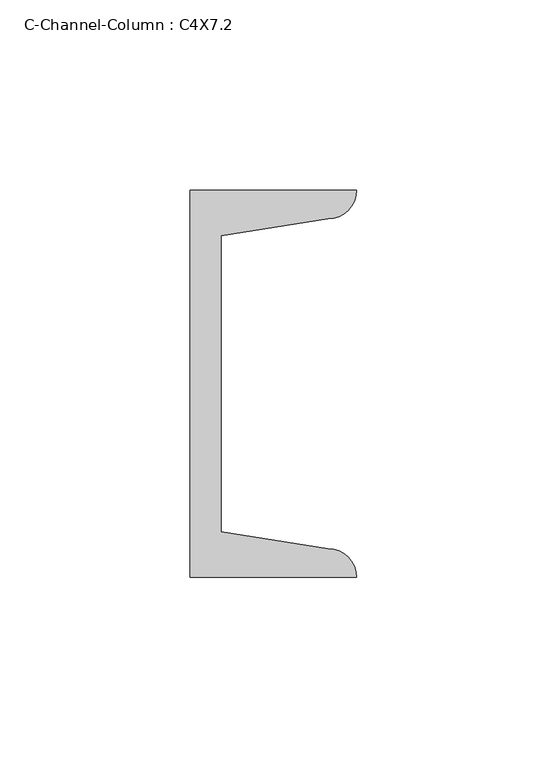
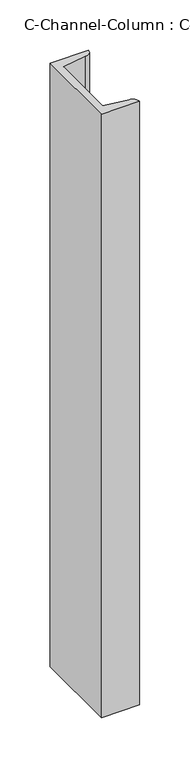
"""IFC4 building model written with IfcOpenShell, lengths in millimetres: column geometry, C-Channel-Column : C4X7.2."""

from ifc_helpers import new_model, si_unit, point, frame, frame_2d, origin, place, context, project, spatial, polyline, circle_curve, trimmed, segment, composite_curve, outline, extrude, source, transform, mapped, element, save


def c_channel_column_c4x7_2_edca617f(model_context):
    return source(origin(), model_context, "Body", "SweptSolid", [
        extrude(outline(composite_curve([segment(polyline([(-11.6586, 50.8), (32.0294, 50.8)]), True, "CONTINUOUS"), segment(trimmed(circle_curve(frame_2d((24.511, 50.8)), 7.5184), [point((32.0294, 50.8))], [point((24.511, 43.2816))], False, "CARTESIAN"), True, "CONTINUOUS"), segment(polyline([(24.511, 43.2816), (-3.5052, 38.8442698), (-3.5052, -38.8442698), (24.511, -43.2816)]), True, "CONTINUOUS"), segment(trimmed(circle_curve(frame_2d((24.511, -50.8)), 7.5184), [point((24.511, -43.2816))], [point((32.0294, -50.8))], False, "CARTESIAN"), True, "CONTINUOUS"), segment(polyline([(32.0294, -50.8), (-11.6586, -50.8), (-11.6586, 50.8)]), True, "CONTINUOUS")], self_intersect=False)), frame((0.0, 0.0, 15474.95), z_axis=(0.0, 0.0, 1.0), x_axis=(1.0, 0.0, 0.0)), (0.0, 0.0, 1.0), 730.25),
    ])


if __name__ == "__main__":
    model = new_model("IFC4")
    model_context = context("Model", 3, world=origin())
    ifc_project = project(units=[si_unit("LENGTHUNIT", "METRE", prefix="MILLI")], contexts=[model_context])
    site = spatial("IfcSite", under=ifc_project)
    building = spatial("IfcBuilding", under=site)
    placement = place(None, origin())
    c_channel_column_c4x7_2_shape = c_channel_column_c4x7_2_edca617f(model_context)
    element("IfcColumn", 1, ObjectType="C-Channel-Column : C4X7.2", at=placement, inside=building, context=model_context, shape_type="MappedRepresentation", body=[
        mapped(c_channel_column_c4x7_2_shape, transform((0.0, 0.0, 0.0), x_axis=(1.0, 0.0, 0.0), y_axis=(0.0, 1.0, 0.0), z_axis=(0.0, 0.0, 1.0))),
    ])
    save(model, "model.ifc")

# Revit data of these elements
# Type "C-Channel-Column : C4X7.2"
#   Assembly Code = "B10"
#   x = 0' - 0.459"
#   W = 7.2
#   bf = 0' - 1.72"
#   d = 0' - 4"
#   tf = 0' - 0.296"
#   tw = 0' - 0.321"
#   A = 0.0147917 SF
#   Structural Material [instance default] = Steel ASTM A36
# Element 1 (IfcColumn, "C-Channel-Column : C4X7.2")
#   Materials on its faces: "Steel ASTM A36"
# Materials
#   "Steel ASTM A36": class "Metal", colour RGB 199 199 199, transparency 0, Description = "Structural steel, ASTM A36 Grade B, mill finish", Cost = 0
